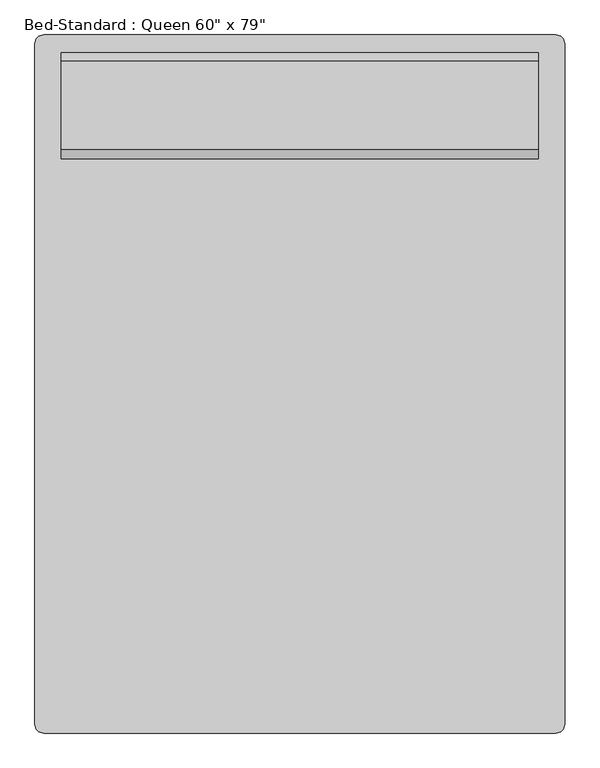
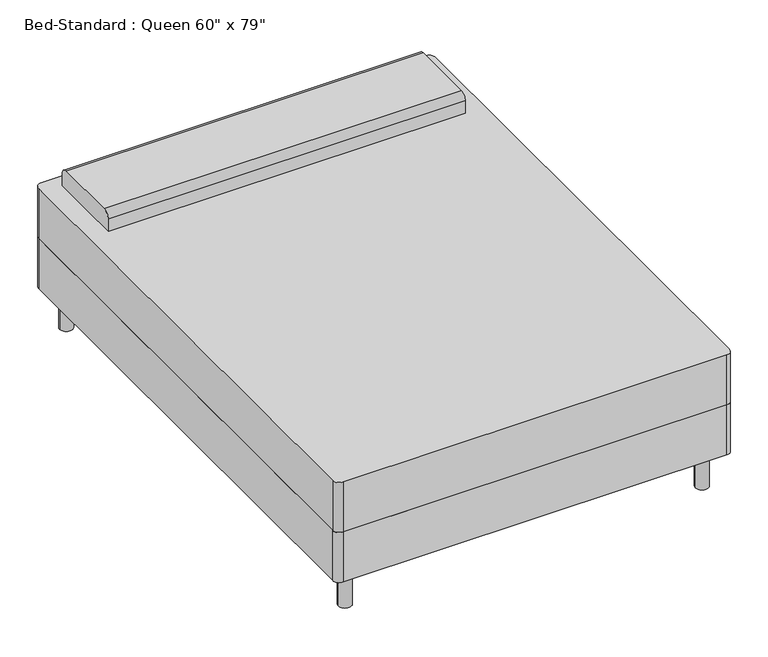
"""IFC4 building model written with IfcOpenShell, lengths in millimetres: furniture geometry."""

import ifcopenshell
import ifcopenshell.guid

model = None  # the IFC model being written
_history = None  # IfcOwnerHistory: only IFC2X3 demands one
_inside = {}  # id of a spatial element -> (the spatial element, [elements in it])
_under = {}  # id of a project, library or spatial element -> (it, [spatial elements below it])
_declared = {}  # id of a project -> (the project, [libraries it declares])
_typed = {}  # id of a type object -> (the type object, [elements of that type])
_made_of = {}  # id of a material, layer set ... -> (it, [elements and type objects made of it])


def new_model(schema):
    """Start an empty IFC model of exactly this schema.

    Asked for "IFC4X3", IfcOpenShell would pick the latest addendum, in which some entities
    have other attributes; the version numbers below select the first issue.
    IFC2X3 requires an IfcOwnerHistory on every rooted entity: one is made here for all.
    """
    global model, _history
    if schema == "IFC4X3":
        model = ifcopenshell.file(schema_version=(4, 3, 0, 0))
    else:
        model = ifcopenshell.file(schema=schema)
    _inside.clear()
    _under.clear()
    _declared.clear()
    _typed.clear()
    _made_of.clear()
    _history = None
    if model.schema == "IFC2X3":
        org = make("IfcOrganization", Name="unknown")
        user = make(
            "IfcPersonAndOrganization",
            ThePerson=make("IfcPerson", FamilyName="unknown"),
            TheOrganization=org,
        )
        app = make(
            "IfcApplication",
            ApplicationDeveloper=org,
            Version="unknown",
            ApplicationFullName="unknown",
            ApplicationIdentifier="unknown",
        )
        _history = make(
            "IfcOwnerHistory",
            OwningUser=user,
            OwningApplication=app,
            ChangeAction="ADDED",
            CreationDate=0,
        )
    return model


def make(cls, **values):
    """One entity of the class cls with the attributes given. An attribute that is None is left unset."""
    return model.create_entity(
        cls, **{name: value for name, value in values.items() if value is not None}
    )


def rooted(cls, **values):
    """An entity with a GlobalId (a new one), such as an element, a storey or a relation."""
    return make(cls, GlobalId=ifcopenshell.guid.new(), OwnerHistory=_history, **values)


def si_unit(unit_type, name, prefix=None):
    """IfcSIUnit, for example si_unit("LENGTHUNIT", "METRE", prefix="MILLI")."""
    return make("IfcSIUnit", UnitType=unit_type, Prefix=prefix, Name=name)


def assignment(units):
    """IfcUnitAssignment: the units of a project."""
    return None if units is None else make("IfcUnitAssignment", Units=units)


def point(xyz):
    """IfcCartesianPoint."""
    return None if xyz is None else make("IfcCartesianPoint", Coordinates=xyz)


def direction(xyz):
    """IfcDirection."""
    return None if xyz is None else make("IfcDirection", DirectionRatios=xyz)


def frame(location, z_axis=None, x_axis=None):
    """IfcAxis2Placement3D, a coordinate frame: its origin and axes. An axis left out is left unset."""
    return make(
        "IfcAxis2Placement3D",
        Location=point(location),
        Axis=direction(z_axis),
        RefDirection=direction(x_axis),
    )


def frame_2d(location, x_axis=None):
    """IfcAxis2Placement2D, a coordinate frame in the plane: its origin and x axis."""
    return make(
        "IfcAxis2Placement2D", Location=point(location), RefDirection=direction(x_axis)
    )


def origin():
    """The frame at (0, 0, 0) with its axes left unset."""
    return frame((0.0, 0.0, 0.0))


def origin_with_axes():
    """The frame at (0, 0, 0) with the z axis (0, 0, 1) and the x axis (1, 0, 0) written out."""
    return frame((0.0, 0.0, 0.0), z_axis=(0.0, 0.0, 1.0), x_axis=(1.0, 0.0, 0.0))


def place(relative_to, where):
    """IfcLocalPlacement: puts the frame where relative to a parent placement (None: the world)."""
    return make(
        "IfcLocalPlacement", PlacementRelTo=relative_to, RelativePlacement=where
    )


def context(
    kind, dimensions, precision=None, world=None, true_north=None, identifier=None
):
    """IfcGeometricRepresentationContext, for example the 3D "Model" context."""
    return make(
        "IfcGeometricRepresentationContext",
        ContextIdentifier=identifier,
        ContextType=kind,
        CoordinateSpaceDimension=dimensions,
        Precision=precision,
        WorldCoordinateSystem=world,
        TrueNorth=true_north,
    )


def project(units=None, contexts=None):
    """IfcProject with its units and contexts."""
    return rooted(
        "IfcProject",
        Name="project",
        RepresentationContexts=contexts,
        UnitsInContext=assignment(units),
    )


def spatial(cls, under=None, at=None, **own):
    """A site, building, storey or space (cls), placed at a placement, below another one or the project."""
    s = rooted(cls, ObjectPlacement=at, **own)
    if under is not None:
        _under.setdefault(under.id(), (under, []))[1].append(s)
    return s


def polyline(points):
    """IfcPolyline through the points."""
    return make("IfcPolyline", Points=[point(p) for p in points])


def circle_curve(where, radius):
    """IfcCircle in the frame where."""
    return make("IfcCircle", Position=where, Radius=radius)


def trimmed(basis, trim1, trim2, sense, master):
    """IfcTrimmedCurve: the piece of a basis curve between two trims."""
    return make(
        "IfcTrimmedCurve",
        BasisCurve=basis,
        Trim1=trim1,
        Trim2=trim2,
        SenseAgreement=sense,
        MasterRepresentation=master,
    )


def segment(curve, same_sense, transition):
    """IfcCompositeCurveSegment."""
    return make(
        "IfcCompositeCurveSegment",
        Transition=transition,
        SameSense=same_sense,
        ParentCurve=curve,
    )


def composite_curve(segments, self_intersect=None):
    """IfcCompositeCurve: segments joined end to end."""
    return make("IfcCompositeCurve", Segments=segments, SelfIntersect=self_intersect)


def outline(outer, holes=None, kind="AREA"):
    """IfcArbitraryClosedProfileDef: a profile drawn as a closed curve; with holes, ...WithVoids."""
    if holes is None:
        return make("IfcArbitraryClosedProfileDef", ProfileType=kind, OuterCurve=outer)
    return make(
        "IfcArbitraryProfileDefWithVoids",
        ProfileType=kind,
        OuterCurve=outer,
        InnerCurves=holes,
    )


def extrude(swept, where, along, depth):
    """IfcExtrudedAreaSolid: the profile swept, set in the frame where, extruded along a direction by depth."""
    return make(
        "IfcExtrudedAreaSolid",
        SweptArea=swept,
        Position=where,
        ExtrudedDirection=direction(along),
        Depth=depth,
    )


def shape(context_of_items, identifier, shape_type, items):
    """IfcShapeRepresentation: the items that make up one representation, for example the "Body"."""
    return make(
        "IfcShapeRepresentation",
        ContextOfItems=context_of_items,
        RepresentationIdentifier=identifier,
        RepresentationType=shape_type,
        Items=items,
    )


def source(mapping_origin, context_of_items, identifier, shape_type, items):
    """IfcRepresentationMap: a shape defined once, which mapped items show again and again."""
    return make(
        "IfcRepresentationMap",
        MappingOrigin=mapping_origin,
        MappedRepresentation=shape(context_of_items, identifier, shape_type, items),
    )


def transform(
    local_origin,
    x_axis=None,
    y_axis=None,
    z_axis=None,
    scale=None,
    scale2=None,
    scale3=None,
    uniform=True,
):
    """IfcCartesianTransformationOperator3D, or its non-uniform kind. x_axis, y_axis, z_axis: its Axis1, 2, 3."""
    if uniform:
        return make(
            "IfcCartesianTransformationOperator3D",
            Axis1=direction(x_axis),
            Axis2=direction(y_axis),
            LocalOrigin=point(local_origin),
            Scale=scale,
            Axis3=direction(z_axis),
        )
    return make(
        "IfcCartesianTransformationOperator3DnonUniform",
        Axis1=direction(x_axis),
        Axis2=direction(y_axis),
        LocalOrigin=point(local_origin),
        Scale=scale,
        Axis3=direction(z_axis),
        Scale2=scale2,
        Scale3=scale3,
    )


def mapped(mapping_source, mapping_target):
    """IfcMappedItem: shows the shape of a source again, moved by a transform."""
    return make(
        "IfcMappedItem", MappingSource=mapping_source, MappingTarget=mapping_target
    )


def made_of(thing, what):
    """Note that an element or type object is made of a material, layer set ...; save() writes the relation."""
    if what is not None:
        _made_of.setdefault(what.id(), (what, []))[1].append(thing)
    return thing


def element(
    cls,
    number,
    at=None,
    inside=None,
    cuts=None,
    type_object=None,
    material=None,
    context=None,
    identifier="Body",
    shape_type=None,
    held_by="IfcProductDefinitionShape",
    body=None,
    shapes=None,
    **own,
):
    """One element of the class cls, such as IfcWall. Its Tag is "e" and its number.

    at: its placement. inside: the storey or other place that contains it. cuts: it is an
    opening in that element (IfcRelVoidsElement). A single representation is given by context,
    identifier, shape_type and body (its items); several are given by shapes. held_by: the class
    of the entity that holds the representations. save() writes the other relations.
    """
    e = rooted(cls, Tag="e%d" % number, ObjectPlacement=at, **own)
    if body is not None:
        shapes = [shape(context, identifier, shape_type, body)]
    if shapes is not None:
        e.Representation = make(held_by, Representations=shapes)
    if inside is not None:
        _inside.setdefault(inside.id(), (inside, []))[1].append(e)
    if cuts is not None:
        rooted(
            "IfcRelVoidsElement", RelatingBuildingElement=cuts, RelatedOpeningElement=e
        )
    if type_object is not None:
        _typed.setdefault(type_object.id(), (type_object, []))[1].append(e)
    return made_of(e, material)


def aggregate(whole, parts):
    """IfcRelAggregates: a whole, such as a stair, and the parts it consists of."""
    return rooted("IfcRelAggregates", RelatingObject=whole, RelatedObjects=parts)


def save(model, path):
    """Write the relations noted so far, then the file.

    IfcRelAggregates (storeys below a building ...), IfcRelContainedInSpatialStructure (elements
    in a storey), IfcRelDefinesByType, IfcRelAssociatesMaterial and IfcRelDeclares: one each for
    every whole, place, type object, material and project.
    """
    for whole, parts in _under.values():
        aggregate(whole, parts)
    for where, things in _inside.values():
        rooted(
            "IfcRelContainedInSpatialStructure",
            RelatedElements=things,
            RelatingStructure=where,
        )
    for kind, things in _typed.values():
        rooted("IfcRelDefinesByType", RelatedObjects=things, RelatingType=kind)
    for what, things in _made_of.values():
        rooted("IfcRelAssociatesMaterial", RelatedObjects=things, RelatingMaterial=what)
    for by, libraries in _declared.values():
        rooted("IfcRelDeclares", RelatingContext=by, RelatedDefinitions=libraries)
    model.write(path)


def furniture_e1791683(model_context):
    return source(origin(), model_context, "Body", "SweptSolid", [
        extrude(outline(composite_curve([segment(polyline([(-490.5114754, -1023.495082), (-490.5114754, 932.304918)]), True, "CONTINUOUS"), segment(trimmed(circle_curve(frame_2d((-465.1114754, 932.304918)), 25.4), [point((-490.5114754, 932.304918))], [point((-465.1114754, 957.704918))], False, "CARTESIAN"), True, "CONTINUOUS"), segment(polyline([(-465.1114754, 957.704918), (1008.0885246, 957.704918)]), True, "CONTINUOUS"), segment(trimmed(circle_curve(frame_2d((1008.0885246, 932.304918)), 25.4), [point((1008.0885246, 957.704918))], [point((1033.4885246, 932.304918))], False, "CARTESIAN"), True, "CONTINUOUS"), segment(polyline([(1033.4885246, 932.304918), (1033.4885246, -1023.495082)]), True, "CONTINUOUS"), segment(trimmed(circle_curve(frame_2d((1008.0885246, -1023.495082)), 25.4), [point((1033.4885246, -1023.495082))], [point((1008.0885246, -1048.895082))], False, "CARTESIAN"), True, "CONTINUOUS"), segment(polyline([(1008.0885246, -1048.895082), (-465.1114754, -1048.895082)]), True, "CONTINUOUS"), segment(trimmed(circle_curve(frame_2d((-465.1114754, -1023.495082)), 25.4), [point((-465.1114754, -1048.895082))], [point((-490.5114754, -1023.495082))], False, "CARTESIAN"), True, "CONTINUOUS")], self_intersect=False)), frame((0.0, 0.0, 152.4), z_axis=(0.0, 0.0, 1.0), x_axis=(1.0, 0.0, 0.0)), (0.0, 0.0, 1.0), 203.2),
        extrude(outline(composite_curve([segment(polyline([(602.104918, 558.8), (602.104918, 609.6)]), True, "CONTINUOUS"), segment(trimmed(circle_curve(frame_2d((627.504918, 609.6)), 25.4), [point((602.104918, 609.6))], [point((627.504918, 635.0))], False, "CARTESIAN"), True, "CONTINUOUS"), segment(polyline([(627.504918, 635.0), (881.504918, 635.0)]), True, "CONTINUOUS"), segment(trimmed(circle_curve(frame_2d((881.504918, 609.6)), 25.4), [point((881.504918, 635.0))], [point((906.904918, 609.6))], False, "CARTESIAN"), True, "CONTINUOUS"), segment(polyline([(906.904918, 609.6), (906.904918, 558.8), (602.104918, 558.8)]), True, "CONTINUOUS")], self_intersect=False)), frame((-414.3114754, 0.0, 0.0), z_axis=(1.0, 0.0, 0.0), x_axis=(0.0, 1.0, 0.0)), (0.0, 0.0, 1.0), 1371.6),
        extrude(outline(composite_curve([segment(trimmed(circle_curve(frame_2d((-414.3114754, 881.504918)), 25.4), [point((-439.7114754, 881.504918))], [point((-388.9114754, 881.504918))], False, "CARTESIAN"), True, "CONTINUOUS"), segment(trimmed(circle_curve(frame_2d((-414.3114754, 881.504918)), 25.4), [point((-388.9114754, 881.504918))], [point((-439.7114754, 881.504918))], False, "CARTESIAN"), True, "CONTINUOUS")], self_intersect=False)), origin_with_axes(), (0.0, 0.0, 1.0), 152.4),
        extrude(outline(composite_curve([segment(trimmed(circle_curve(frame_2d((957.2885246, 881.504918)), 25.4), [point((931.8885246, 881.504918))], [point((982.6885246, 881.504918))], False, "CARTESIAN"), True, "CONTINUOUS"), segment(trimmed(circle_curve(frame_2d((957.2885246, 881.504918)), 25.4), [point((982.6885246, 881.504918))], [point((931.8885246, 881.504918))], False, "CARTESIAN"), True, "CONTINUOUS")], self_intersect=False)), origin_with_axes(), (0.0, 0.0, 1.0), 152.4),
        extrude(outline(composite_curve([segment(trimmed(circle_curve(frame_2d((957.2885246, -972.695082)), 25.4), [point((931.8885246, -972.695082))], [point((982.6885246, -972.695082))], False, "CARTESIAN"), True, "CONTINUOUS"), segment(trimmed(circle_curve(frame_2d((957.2885246, -972.695082)), 25.4), [point((982.6885246, -972.695082))], [point((931.8885246, -972.695082))], False, "CARTESIAN"), True, "CONTINUOUS")], self_intersect=False)), origin_with_axes(), (0.0, 0.0, 1.0), 152.4),
        extrude(outline(composite_curve([segment(trimmed(circle_curve(frame_2d((-414.3114754, -972.695082)), 25.4), [point((-439.7114754, -972.695082))], [point((-388.9114754, -972.695082))], False, "CARTESIAN"), True, "CONTINUOUS"), segment(trimmed(circle_curve(frame_2d((-414.3114754, -972.695082)), 25.4), [point((-388.9114754, -972.695082))], [point((-439.7114754, -972.695082))], False, "CARTESIAN"), True, "CONTINUOUS")], self_intersect=False)), origin_with_axes(), (0.0, 0.0, 1.0), 152.4),
        extrude(outline(composite_curve([segment(polyline([(-465.1114754, 957.704918), (1008.0885246, 957.704918)]), True, "CONTINUOUS"), segment(trimmed(circle_curve(frame_2d((1008.0885246, 932.304918)), 25.4), [point((1008.0885246, 957.704918))], [point((1033.4885246, 932.304918))], False, "CARTESIAN"), True, "CONTINUOUS"), segment(polyline([(1033.4885246, 932.304918), (1033.4885246, -1023.495082)]), True, "CONTINUOUS"), segment(trimmed(circle_curve(frame_2d((1008.0885246, -1023.495082)), 25.4), [point((1033.4885246, -1023.495082))], [point((1008.0885246, -1048.895082))], False, "CARTESIAN"), True, "CONTINUOUS"), segment(polyline([(1008.0885246, -1048.895082), (-465.1114754, -1048.895082)]), True, "CONTINUOUS"), segment(trimmed(circle_curve(frame_2d((-465.1114754, -1023.495082)), 25.4), [point((-465.1114754, -1048.895082))], [point((-490.5114754, -1023.495082))], False, "CARTESIAN"), True, "CONTINUOUS"), segment(polyline([(-490.5114754, -1023.495082), (-490.5114754, 932.304918)]), True, "CONTINUOUS"), segment(trimmed(circle_curve(frame_2d((-465.1114754, 932.304918)), 25.4), [point((-490.5114754, 932.304918))], [point((-465.1114754, 957.704918))], False, "CARTESIAN"), True, "CONTINUOUS")], self_intersect=False)), frame((0.0, 0.0, 355.6), z_axis=(0.0, 0.0, 1.0), x_axis=(1.0, 0.0, 0.0)), (0.0, 0.0, 1.0), 203.2),
    ])


if __name__ == "__main__":
    model = new_model("IFC4")
    model_context = context("Model", 3, world=origin())
    ifc_project = project(units=[si_unit("LENGTHUNIT", "METRE", prefix="MILLI")], contexts=[model_context])
    site = spatial("IfcSite", under=ifc_project)
    building = spatial("IfcBuilding", under=site)
    placement = place(None, origin())
    furniture_shape = furniture_e1791683(model_context)
    element("IfcFurniture", 1, ObjectType="Bed-Standard : Queen 60\" x 79\"", at=placement, inside=building, context=model_context, shape_type="MappedRepresentation", body=[
        mapped(furniture_shape, transform((0.0, 0.0, 0.0), x_axis=(1.0, 0.0, 0.0), y_axis=(0.0, 1.0, 0.0), z_axis=(0.0, 0.0, 1.0))),
    ])
    save(model, "model.ifc")

# Revit data of these elements
# Type "Bed-Standard : Queen 60\" x 79\""
#   Assembly Code = "E2020200"
#   Clear Dim_2 = 2' - 0"
#   Clear Dim_1 = 3' - 0"
#   Length = 6' - 7"
#   Width = 5' - 0"
#   Leg Material = Metal - Chrome
#   Mattress Material = Textile - White
# Element 1 (IfcFurniture, "Bed-Standard : Queen 60\" x 79\"")
#   Materials on its faces: "Textile - White", "Metal - Chrome"
# Materials
#   "Metal - Chrome": class "Metal", colour RGB 17 17 17, transparency 0
#   "Textile - White": class "Fabric", colour RGB 247 247 239, transparency 0
